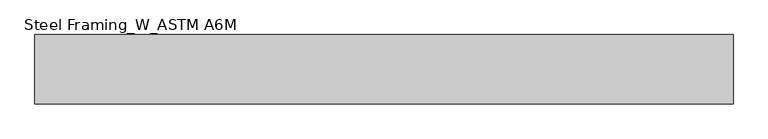
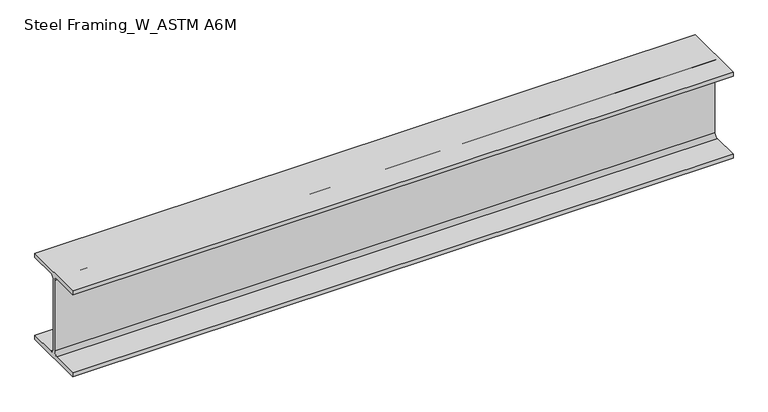
"""IFC4 building model written with IfcOpenShell, lengths in millimetres: beam geometry, Steel Framing_W_ASTM A6M : H_SB_AR_S02_W360x91_B3."""

from ifc_helpers import new_model, si_unit, point, frame, frame_2d, origin, place, context, project, spatial, polyline, circle_curve, trimmed, segment, composite_curve, outline, extrude, source, transform, mapped, element, save


def steel_framing_w_astm_a6m_a9de8b5d(model_context):
    return source(origin(), model_context, "Body", "SweptSolid", [
        extrude(outline(composite_curve([segment(polyline([(127.0, -160.1), (127.0, -176.5), (-127.0, -176.5), (-127.0, -160.1), (-19.865, -160.1)]), True, "CONTINUOUS"), segment(trimmed(circle_curve(frame_2d((-19.865, -145.0)), 15.1), [point((-19.865, -160.1))], [point((-4.765, -145.0))], True, "CARTESIAN"), True, "CONTINUOUS"), segment(polyline([(-4.765, -145.0), (-4.765, 145.0)]), True, "CONTINUOUS"), segment(trimmed(circle_curve(frame_2d((-19.865, 145.0)), 15.1), [point((-4.765, 145.0))], [point((-19.865, 160.1))], True, "CARTESIAN"), True, "CONTINUOUS"), segment(polyline([(-19.865, 160.1), (-127.0, 160.1), (-127.0, 176.5), (127.0, 176.5), (127.0, 160.1), (19.865, 160.1)]), True, "CONTINUOUS"), segment(trimmed(circle_curve(frame_2d((19.865, 145.0)), 15.1), [point((19.865, 160.1))], [point((4.765, 145.0))], True, "CARTESIAN"), True, "CONTINUOUS"), segment(polyline([(4.765, 145.0), (4.765, -145.0)]), True, "CONTINUOUS"), segment(trimmed(circle_curve(frame_2d((19.865, -145.0)), 15.1), [point((4.765, -145.0))], [point((19.865, -160.1))], True, "CARTESIAN"), True, "CONTINUOUS"), segment(polyline([(19.865, -160.1), (127.0, -160.1)]), True, "CONTINUOUS")], self_intersect=False)), frame((-1203.3, 0.0, 0.0), z_axis=(1.0, 0.0, 0.0), x_axis=(0.0, 1.0, 0.0)), (0.0, 0.0, 1.0), 2563.6),
    ])


if __name__ == "__main__":
    model = new_model("IFC4")
    model_context = context("Model", 3, world=origin())
    ifc_project = project(units=[si_unit("LENGTHUNIT", "METRE", prefix="MILLI")], contexts=[model_context])
    site = spatial("IfcSite", under=ifc_project)
    building = spatial("IfcBuilding", under=site)
    placement = place(None, origin())
    steel_framing_w_astm_a6m_shape = steel_framing_w_astm_a6m_a9de8b5d(model_context)
    element("IfcBeam", 1, ObjectType="Steel Framing_W_ASTM A6M : H_SB_AR_S02_W360x91_B3", at=placement, inside=building, context=model_context, shape_type="MappedRepresentation", body=[
        mapped(steel_framing_w_astm_a6m_shape, transform((0.0, 0.0, 0.0), x_axis=(1.0, 0.0, 0.0), y_axis=(0.0, 1.0, 0.0), z_axis=(0.0, 0.0, 1.0))),
    ])
    save(model, "model.ifc")

# Revit data of these elements
# Type "Steel Framing_W_ASTM A6M : H_SB_AR_S02_W360x91_B3"
#   Type Mark = "B3"
#   Section Name Key = "W14x61"
#   Width = 25.4 cm
#   Web Thickness = 0.953 cm
#   Web Fillet = 1.51 cm
#   Warping Constant = 1260000.0 cm⁶
#   Torsional Moment of Inertia = 91.20 cm⁴
#   Section Area = 115.0 cm²
#   Plastic Modulus weak axis = 537.0 cm³
#   Plastic Modulus strong axis = 1670.0 cm³
#   Perimeter = 1.68 m²/m
#   Nominal Weight = 91.00 kgf/m
#   Moment of Inertia weak axis = 4450.00 cm⁴
#   Moment of Inertia strong axis = 26600.00 cm⁴
#   Height = 35.3 cm
#   Flange Thickness = 1.64 cm
#   Elastic Modulus weak axis = 352.0 cm³
#   Elastic Modulus strong axis = 1510.0 cm³
#   Centroid Vertical = 17.65 cm
#   Centroid Horizontal = 12.7 cm
#   Length [instance default] = 1500 mm
#   Structural Material [instance default] = Steel, 45-345
#   Bolt Spacing = 0
#   Assembly Code = ""
# Element 1 (IfcBeam, "Steel Framing_W_ASTM A6M : H_SB_AR_S02_W360x91_B3")
#   Materials on its faces: "Steel, 45-345"
# Materials
#   "Steel, 45-345": class "Metal", colour RGB 189 187 185, transparency 0, Description = "Steel 345 MPa", Cost = 0
